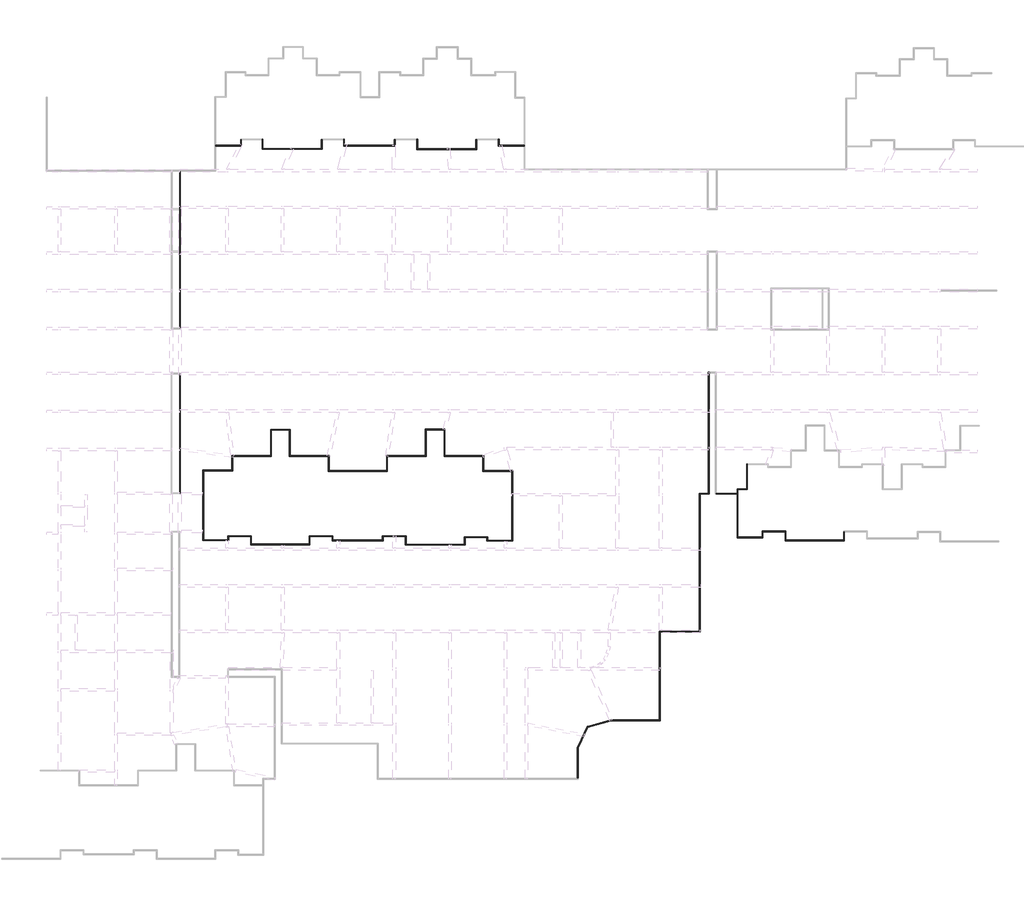
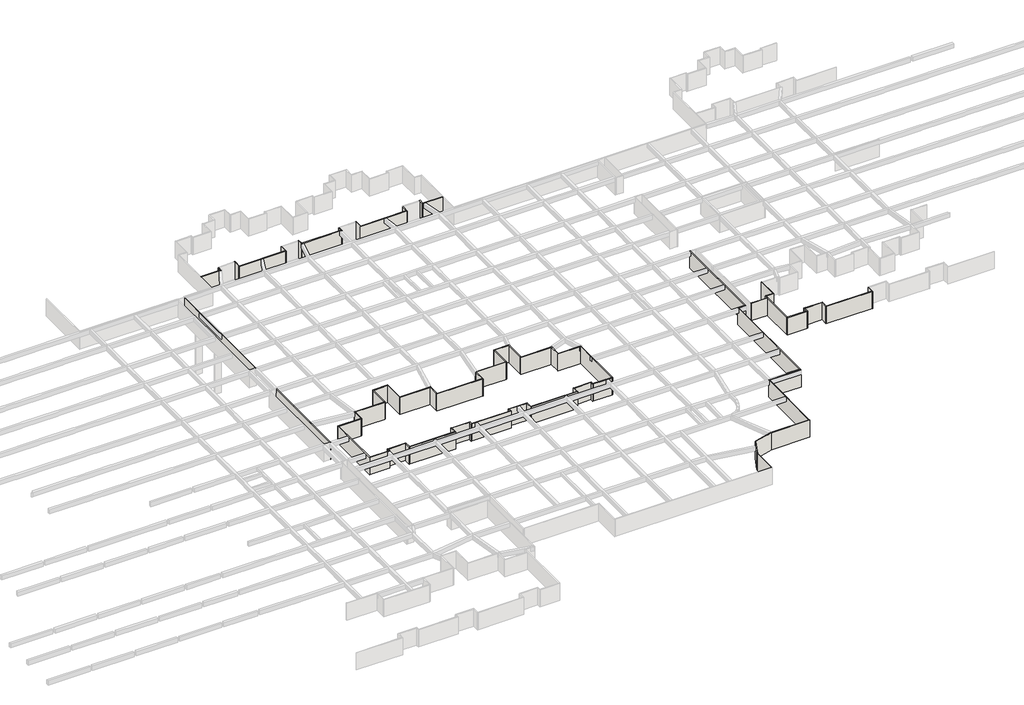
# One storey, part 4 of 16: 70 walls.
"""IFC4 building model written with IfcOpenShell, lengths in millimetres."""

from ifc_helpers import new_model, si_unit, origin, origin_with_axes, place, context, project, spatial, polyline, outline, extrude, faceted_brep, element, save

model = new_model("IFC4")

# Units and contexts
model_context = context("Model", 3, world=origin())
ifc_project = project(units=[si_unit("LENGTHUNIT", "METRE", prefix="MILLI")], contexts=[model_context])

# Site, building, storey
site = spatial("IfcSite", under=ifc_project)
building = spatial("IfcBuilding", under=site)
storey = spatial("IfcBuildingStorey", under=building, Name="户型图", Elevation=0.0)

# Walls
placement = place(None, origin())
element("IfcWall", 1, ObjectType="所有墙体", at=placement, inside=storey, context=model_context, shape_type="Brep", body=[
    faceted_brep([(305606.5285699, -128840.8246701, 0.0), (302019.0558962, -128840.8246701, 0.0), (301899.0558962, -128840.8246701, 0.0), (301899.0558962, -128840.8246701, 3300.0), (302019.0558962, -128840.8246701, 3300.0), (305606.5285699, -128840.8246701, 3300.0), (305606.5285699, -128960.8246701, 0.0), (305606.5285699, -128960.8246701, 3300.0), (301899.0558962, -128960.8246701, 3300.0), (301899.0558962, -128960.8246701, 0.0)], [[[0, 1, 2, 3, 4, 5]], [[6, 7, 8, 9]], [[2, 1, 0, 6, 9]], [[5, 4, 3, 8, 7]], [[0, 5, 7, 6]], [[3, 2, 9, 8]]]),
])
element("IfcWall", 2, ObjectType="所有墙体", at=placement, inside=storey, context=model_context, shape_type="Brep", body=[
    faceted_brep([(302019.0558962, -128840.8246701, 0.0), (302019.0558962, -127937.9986276, 0.0), (302019.0558962, -127937.9986276, 3300.0), (302019.0558962, -128840.8246701, 3300.0), (301899.0558962, -128840.8246701, 0.0), (301899.0558962, -128840.8246701, 3300.0), (301899.0558962, -128057.9986276, 3300.0), (301899.0558962, -127937.9986276, 3300.0), (301899.0558962, -127937.9986276, 0.0), (301899.0558962, -128057.9986276, 0.0)], [[[0, 1, 2, 3]], [[4, 5, 6, 7, 8, 9]], [[1, 0, 4, 9, 8]], [[3, 2, 7, 6, 5]], [[0, 3, 5, 4]], [[2, 1, 8, 7]]]),
])
element("IfcWall", 3, ObjectType="所有墙体", at=placement, inside=storey, context=model_context, shape_type="Brep", body=[
    faceted_brep([(298699.7203632, -128057.9986276, 0.0), (298699.7203632, -129334.4293697, 0.0), (298699.7203632, -129454.4293697, 0.0), (298699.7203632, -129454.4293697, 3300.0), (298699.7203632, -129334.4293697, 3300.0), (298699.7203632, -128057.9986276, 3300.0), (298819.7203632, -128057.9986276, 0.0), (298819.7203632, -128057.9986276, 3300.0), (298819.7203632, -129454.4293697, 3300.0), (298819.7203632, -129454.4293697, 0.0)], [[[0, 1, 2, 3, 4, 5]], [[6, 7, 8, 9]], [[2, 1, 0, 6, 9]], [[5, 4, 3, 8, 7]], [[0, 5, 7, 6]], [[3, 2, 9, 8]]]),
])
element("IfcWall", 4, ObjectType="所有墙体", at=placement, inside=storey, context=model_context, shape_type="Brep", body=[
    faceted_brep([(298699.7203632, -129334.4293697, 0.0), (290319.7203632, -129334.4293697, 0.0), (290199.7203632, -129334.4293697, 0.0), (290199.7203632, -129334.4293697, 3300.0), (290319.7203632, -129334.4293697, 3300.0), (298699.7203632, -129334.4293697, 3300.0), (298699.7203632, -129454.4293697, 0.0), (298699.7203632, -129454.4293697, 3300.0), (290199.7203632, -129454.4293697, 3300.0), (290199.7203632, -129454.4293697, 0.0)], [[[0, 1, 2, 3, 4, 5]], [[6, 7, 8, 9]], [[2, 1, 0, 6, 9]], [[5, 4, 3, 8, 7]], [[0, 5, 7, 6]], [[3, 2, 9, 8]]]),
])
element("IfcWall", 5, ObjectType="所有墙体", at=placement, inside=storey, context=model_context, shape_type="Brep", body=[
    faceted_brep([(290319.7203632, -129334.4293697, 0.0), (290319.7203632, -127937.9986276, 0.0), (290319.7203632, -127937.9986276, 3300.0), (290319.7203632, -129334.4293697, 3300.0), (290199.7203632, -129334.4293697, 0.0), (290199.7203632, -129334.4293697, 3300.0), (290199.7203632, -128057.9986276, 3300.0), (290199.7203632, -127937.9986276, 3300.0), (290199.7203632, -127937.9986276, 0.0), (290199.7203632, -128057.9986276, 0.0)], [[[0, 1, 2, 3]], [[4, 5, 6, 7, 8, 9]], [[1, 0, 4, 9, 8]], [[3, 2, 7, 6, 5]], [[0, 3, 5, 4]], [[2, 1, 8, 7]]]),
])
element("IfcWall", 6, ObjectType="所有墙体", at=placement, inside=storey, context=model_context, shape_type="Brep", body=[
    faceted_brep([(286999.7203632, -128057.9986276, 0.0), (286999.7203632, -128840.8246701, 0.0), (286999.7203632, -128960.8246701, 0.0), (286999.7203632, -128960.8246701, 3300.0), (286999.7203632, -128840.8246701, 3300.0), (286999.7203632, -128057.9986276, 3300.0), (287119.7203632, -128057.9986276, 0.0), (287119.7203632, -128057.9986276, 3300.0), (287119.7203632, -128960.8246701, 3300.0), (287119.7203632, -128960.8246701, 0.0)], [[[0, 1, 2, 3, 4, 5]], [[6, 7, 8, 9]], [[2, 1, 0, 6, 9]], [[5, 4, 3, 8, 7]], [[0, 5, 7, 6]], [[3, 2, 9, 8]]]),
])
element("IfcWall", 7, ObjectType="所有墙体", at=placement, inside=storey, context=model_context, shape_type="Brep", body=[
    faceted_brep([(286999.7203632, -128840.8246701, 0.0), (279819.0680425, -128840.8246701, 0.0), (279699.0680425, -128840.8246701, 0.0), (279699.0680425, -128840.8246701, 3300.0), (279819.0680425, -128840.8246701, 3300.0), (286999.7203632, -128840.8246701, 3300.0), (286999.7203632, -128960.8246701, 0.0), (286999.7203632, -128960.8246701, 3300.0), (279699.0680425, -128960.8246701, 3300.0), (279699.0680425, -128960.8246701, 0.0)], [[[0, 1, 2, 3, 4, 5]], [[6, 7, 8, 9]], [[2, 1, 0, 6, 9]], [[5, 4, 3, 8, 7]], [[0, 5, 7, 6]], [[3, 2, 9, 8]]]),
])
element("IfcWall", 8, ObjectType="所有墙体", at=placement, inside=storey, context=model_context, shape_type="Brep", body=[
    faceted_brep([(279819.0680425, -128840.8246701, 0.0), (279819.0680425, -127937.9986276, 0.0), (279819.0680425, -127937.9986276, 3300.0), (279819.0680425, -128840.8246701, 3300.0), (279699.0680425, -128840.8246701, 0.0), (279699.0680425, -128840.8246701, 3300.0), (279699.0680425, -128057.9986276, 3300.0), (279699.0680425, -127937.9986276, 3300.0), (279699.0680425, -127937.9986276, 0.0), (279699.0680425, -128057.9986276, 0.0)], [[[0, 1, 2, 3]], [[4, 5, 6, 7, 8, 9]], [[1, 0, 4, 9, 8]], [[3, 2, 7, 6, 5]], [[0, 3, 5, 4]], [[2, 1, 8, 7]]]),
])
element("IfcWall", 9, ObjectType="所有墙体", at=placement, inside=storey, context=model_context, shape_type="Brep", body=[
    faceted_brep([(276499.7065412, -128057.9986276, 0.0), (276499.7065412, -129309.6564364, 0.0), (276499.7065412, -129429.6564364, 0.0), (276499.7065412, -129429.6564364, 3300.0), (276499.7065412, -129309.6564364, 3300.0), (276499.7065412, -128057.9986276, 3300.0), (276619.7065412, -128057.9986276, 0.0), (276619.7065412, -128057.9986276, 3300.0), (276619.7065412, -129429.6564364, 3300.0), (276619.7065412, -129429.6564364, 0.0)], [[[0, 1, 2, 3, 4, 5]], [[6, 7, 8, 9]], [[2, 1, 0, 6, 9]], [[5, 4, 3, 8, 7]], [[0, 5, 7, 6]], [[3, 2, 9, 8]]]),
])
element("IfcWall", 10, ObjectType="所有墙体", at=placement, inside=storey, context=model_context, shape_type="Brep", body=[
    faceted_brep([(276499.7065412, -129309.6564364, 0.0), (268118.1706199, -129309.6564364, 0.0), (267998.1706199, -129309.6564364, 0.0), (267998.1706199, -129309.6564364, 3300.0), (268118.1706199, -129309.6564364, 3300.0), (276499.7065412, -129309.6564364, 3300.0), (276499.7065412, -129429.6564364, 0.0), (276499.7065412, -129429.6564364, 3300.0), (267998.1706199, -129429.6564364, 3300.0), (267998.1706199, -129429.6564364, 0.0)], [[[0, 1, 2, 3, 4, 5]], [[6, 7, 8, 9]], [[2, 1, 0, 6, 9]], [[5, 4, 3, 8, 7]], [[0, 5, 7, 6]], [[3, 2, 9, 8]]]),
])
element("IfcWall", 11, ObjectType="所有墙体", at=placement, inside=storey, context=model_context, shape_type="Brep", body=[
    faceted_brep([(268118.1706199, -129309.6564364, 0.0), (268118.1706199, -127937.9986276, 0.0), (268118.1706199, -127937.9986276, 3300.0), (268118.1706199, -129309.6564364, 3300.0), (267998.1706199, -129309.6564364, 0.0), (267998.1706199, -129309.6564364, 3300.0), (267998.1706199, -128057.9986276, 3300.0), (267998.1706199, -127937.9986276, 3300.0), (267998.1706199, -127937.9986276, 0.0), (267998.1706199, -128057.9986276, 0.0)], [[[0, 1, 2, 3]], [[4, 5, 6, 7, 8, 9]], [[1, 0, 4, 9, 8]], [[3, 2, 7, 6, 5]], [[0, 3, 5, 4]], [[2, 1, 8, 7]]]),
])
element("IfcWall", 12, ObjectType="所有墙体", at=placement, inside=storey, context=model_context, shape_type="Brep", body=[
    faceted_brep([(264899.6993188, -128057.9986276, 0.0), (264899.6993188, -128840.8246701, 0.0), (264899.6993188, -128960.8246701, 0.0), (264899.6993188, -128960.8246701, 3300.0), (264899.6993188, -128840.8246701, 3300.0), (264899.6993188, -128057.9986276, 3300.0), (265019.6993188, -128057.9986276, 0.0), (265019.6993188, -128057.9986276, 3300.0), (265019.6993188, -128960.8246701, 3300.0), (265019.6993188, -128960.8246701, 0.0)], [[[0, 1, 2, 3, 4, 5]], [[6, 7, 8, 9]], [[2, 1, 0, 6, 9]], [[5, 4, 3, 8, 7]], [[0, 5, 7, 6]], [[3, 2, 9, 8]]]),
])
element("IfcWall", 13, ObjectType="所有墙体", at=placement, inside=storey, context=model_context, shape_type="SweptSolid", body=[
    extrude(outline(polyline([(261322.7517568, -128840.8246701), (264899.6993188, -128840.8246701), (264899.6993188, -128960.8246701), (261322.7517568, -128960.8246701), (261322.7517568, -128840.8246701)])), origin_with_axes(), (0.0, 0.0, 1.0), 3300.0),
])
element("IfcWall", 14, ObjectType="所有墙体", at=placement, inside=storey, context=model_context, shape_type="Brep", body=[
    faceted_brep([(351498.9314816, -184368.2301972, 0.0), (351498.9314816, -185539.8859396, 0.0), (351498.9314816, -185659.8859396, 0.0), (351498.9314816, -185659.8859396, 3300.0), (351498.9314816, -185539.8859396, 3300.0), (351498.9314816, -184368.2301972, 3300.0), (351618.9314816, -184368.2301972, 0.0), (351618.9314816, -184368.2301972, 3300.0), (351618.9314816, -185659.8859396, 3300.0), (351618.9314816, -185659.8859396, 0.0)], [[[0, 1, 2, 3, 4, 5]], [[6, 7, 8, 9]], [[2, 1, 0, 6, 9]], [[5, 4, 3, 8, 7]], [[0, 5, 7, 6]], [[3, 2, 9, 8]]]),
])
element("IfcWall", 15, ObjectType="所有墙体", at=placement, inside=storey, context=model_context, shape_type="Brep", body=[
    faceted_brep([(351498.9314816, -185539.8859396, 0.0), (343215.8107635, -185539.8859396, 0.0), (343095.8107635, -185539.8859396, 0.0), (343095.8107635, -185539.8859396, 3300.0), (343215.8107635, -185539.8859396, 3300.0), (351498.9314816, -185539.8859396, 3300.0), (351498.9314816, -185659.8859396, 0.0), (351498.9314816, -185659.8859396, 3300.0), (343095.8107635, -185659.8859396, 3300.0), (343095.8107635, -185659.8859396, 0.0)], [[[0, 1, 2, 3, 4, 5]], [[6, 7, 8, 9]], [[2, 1, 0, 6, 9]], [[5, 4, 3, 8, 7]], [[0, 5, 7, 6]], [[3, 2, 9, 8]]]),
])
element("IfcWall", 16, ObjectType="所有墙体", at=placement, inside=storey, context=model_context, shape_type="Brep", body=[
    faceted_brep([(343215.8107635, -185539.8859396, 0.0), (343215.8107635, -184248.2301972, 0.0), (343215.8107635, -184248.2301972, 3300.0), (343215.8107635, -185539.8859396, 3300.0), (343095.8107635, -185539.8859396, 0.0), (343095.8107635, -185539.8859396, 3300.0), (343095.8107635, -184368.2301972, 3300.0), (343095.8107635, -184248.2301972, 3300.0), (343095.8107635, -184248.2301972, 0.0), (343095.8107635, -184368.2301972, 0.0)], [[[0, 1, 2, 3]], [[4, 5, 6, 7, 8, 9]], [[1, 0, 4, 9, 8]], [[3, 2, 7, 6, 5]], [[0, 3, 5, 4]], [[2, 1, 8, 7]]]),
])
element("IfcWall", 17, ObjectType="所有墙体", at=placement, inside=storey, context=model_context, shape_type="Brep", body=[
    faceted_brep([(343095.8107635, -184248.2301972, 0.0), (339799.0678646, -184248.2301972, 0.0), (339799.0678646, -184248.2301972, 3300.0), (343095.8107635, -184248.2301972, 3300.0), (343095.8107635, -184368.2301972, 0.0), (343095.8107635, -184368.2301972, 3300.0), (339919.0678646, -184368.2301972, 3300.0), (339799.0678646, -184368.2301972, 3300.0), (339799.0678646, -184368.2301972, 0.0), (339919.0678646, -184368.2301972, 0.0)], [[[0, 1, 2, 3]], [[4, 5, 6, 7, 8, 9]], [[1, 0, 4, 9, 8]], [[3, 2, 7, 6, 5]], [[0, 3, 5, 4]], [[2, 1, 8, 7]]]),
])
element("IfcWall", 18, ObjectType="所有墙体", at=placement, inside=storey, context=model_context, shape_type="Brep", body=[
    faceted_brep([(339799.0678646, -184368.2301972, 0.0), (339799.0678646, -185110.2860694, 0.0), (339799.0678646, -185230.2860694, 0.0), (339799.0678646, -185230.2860694, 3300.0), (339799.0678646, -185110.2860694, 3300.0), (339799.0678646, -184368.2301972, 3300.0), (339919.0678646, -184368.2301972, 0.0), (339919.0678646, -184368.2301972, 3300.0), (339919.0678646, -185230.2860694, 3300.0), (339919.0678646, -185230.2860694, 0.0)], [[[0, 1, 2, 3, 4, 5]], [[6, 7, 8, 9]], [[2, 1, 0, 6, 9]], [[5, 4, 3, 8, 7]], [[0, 5, 7, 6]], [[3, 2, 9, 8]]]),
])
element("IfcWall", 19, ObjectType="所有墙体", at=placement, inside=storey, context=model_context, shape_type="Brep", body=[
    faceted_brep([(339799.0678646, -185110.2860694, 0.0), (336316.8754953, -185110.2860694, 0.0), (336196.8754953, -185110.2860694, 0.0), (336196.8754953, -185110.2860694, 3300.0), (336316.8754953, -185110.2860694, 3300.0), (339799.0678646, -185110.2860694, 3300.0), (339799.0678646, -185230.2860694, 0.0), (339799.0678646, -185230.2860694, 3300.0), (336196.8754953, -185230.2860694, 3300.0), (336196.8754953, -185230.2860694, 0.0)], [[[0, 1, 2, 3, 4, 5]], [[6, 7, 8, 9]], [[2, 1, 0, 6, 9]], [[5, 4, 3, 8, 7]], [[0, 5, 7, 6]], [[3, 2, 9, 8]]]),
])
element("IfcWall", 20, ObjectType="所有墙体", at=placement, inside=storey, context=model_context, shape_type="Brep", body=[
    faceted_brep([(336316.8754953, -185110.2860694, 0.0), (336316.8754953, -178321.3511104, 0.0), (336316.8754953, -178201.3511104, 0.0), (336316.8754953, -178201.3511104, 3300.0), (336316.8754953, -178321.3511104, 3300.0), (336316.8754953, -185110.2860694, 3300.0), (336196.8754953, -185110.2860694, 0.0), (336196.8754953, -185110.2860694, 3300.0), (336196.8754953, -178965.1471774, 3300.0), (336196.8754953, -178845.1471774, 3300.0), (336196.8754953, -178201.3511104, 3300.0), (336196.8754953, -178201.3511104, 0.0), (336196.8754953, -178845.1471774, 0.0), (336196.8754953, -178965.1471774, 0.0)], [[[0, 1, 2, 3, 4, 5]], [[6, 7, 8, 9, 10, 11, 12, 13]], [[2, 1, 0, 6, 13, 12, 11]], [[5, 4, 3, 10, 9, 8, 7]], [[0, 5, 7, 6]], [[3, 2, 11, 10]]]),
])
element("IfcWall", 21, ObjectType="所有墙体", at=placement, inside=storey, context=model_context, shape_type="Brep", body=[
    faceted_brep([(336316.8754953, -178321.3511104, 0.0), (337684.3582015, -178321.3511104, 0.0), (337684.3582015, -178321.3511104, 3300.0), (336316.8754953, -178321.3511104, 3300.0), (336316.8754953, -178201.3511104, 0.0), (336316.8754953, -178201.3511104, 3300.0), (337564.3582015, -178201.3511104, 3300.0), (337684.3582015, -178201.3511104, 3300.0), (337684.3582015, -178201.3511104, 0.0), (337564.3582015, -178201.3511104, 0.0)], [[[0, 1, 2, 3]], [[4, 5, 6, 7, 8, 9]], [[1, 0, 4, 9, 8]], [[3, 2, 7, 6, 5]], [[0, 3, 5, 4]], [[2, 1, 8, 7]]]),
])
element("IfcWall", 22, ObjectType="所有墙体", at=placement, inside=storey, context=model_context, shape_type="Brep", body=[
    faceted_brep([(337684.3582015, -178201.3511104, 0.0), (337684.3582015, -174724.5990482, 0.0), (337684.3582015, -174604.5990482, 0.0), (337684.3582015, -174604.5990482, 3300.0), (337684.3582015, -174724.5990482, 3300.0), (337684.3582015, -178201.3511104, 3300.0), (337564.3582015, -178201.3511104, 0.0), (337564.3582015, -178201.3511104, 3300.0), (337564.3582015, -174604.5990482, 3300.0), (337564.3582015, -174604.5990482, 0.0)], [[[0, 1, 2, 3, 4, 5]], [[6, 7, 8, 9]], [[2, 1, 0, 6, 9]], [[5, 4, 3, 8, 7]], [[0, 5, 7, 6]], [[3, 2, 9, 8]]]),
])
element("IfcWall", 23, ObjectType="所有墙体", at=placement, inside=storey, context=model_context, shape_type="Brep", body=[
    faceted_brep([(303975.2880408, -185704.0117748, 0.0), (303975.2880408, -175584.0117748, 0.0), (303975.2880408, -175584.0117748, 3300.0), (303975.2880408, -185704.0117748, 3300.0), (303855.2880408, -185704.0117748, 0.0), (303855.2880408, -185704.0117748, 3300.0), (303855.2880408, -185584.0117748, 3300.0), (303855.2880408, -175704.0117748, 3300.0), (303855.2880408, -175584.0117748, 3300.0), (303855.2880408, -175584.0117748, 0.0), (303855.2880408, -175704.0117748, 0.0), (303855.2880408, -185584.0117748, 0.0)], [[[0, 1, 2, 3]], [[4, 5, 6, 7, 8, 9, 10, 11]], [[1, 0, 4, 11, 10, 9]], [[3, 2, 8, 7, 6, 5]], [[2, 1, 9, 8]], [[0, 3, 5, 4]]]),
])
element("IfcWall", 24, ObjectType="所有墙体", at=placement, inside=storey, context=model_context, shape_type="Brep", body=[
    faceted_brep([(303855.2880408, -175584.0117748, 0.0), (299815.2880408, -175584.0117748, 0.0), (299695.2880408, -175584.0117748, 0.0), (299695.2880408, -175584.0117748, 3300.0), (299815.2880408, -175584.0117748, 3300.0), (303855.2880408, -175584.0117748, 3300.0), (303855.2880408, -175704.0117748, 0.0), (303855.2880408, -175704.0117748, 3300.0), (299695.2880408, -175704.0117748, 3300.0), (299695.2880408, -175704.0117748, 0.0)], [[[0, 1, 2, 3, 4, 5]], [[6, 7, 8, 9]], [[2, 1, 0, 6, 9]], [[5, 4, 3, 8, 7]], [[0, 5, 7, 6]], [[3, 2, 9, 8]]]),
])
element("IfcWall", 25, ObjectType="所有墙体", at=placement, inside=storey, context=model_context, shape_type="Brep", body=[
    faceted_brep([(299815.2880408, -175584.0117748, 0.0), (299815.2880408, -173444.0117748, 0.0), (299815.2880408, -173444.0117748, 3300.0), (299815.2880408, -175584.0117748, 3300.0), (299695.2880408, -175584.0117748, 0.0), (299695.2880408, -175584.0117748, 3300.0), (299695.2880408, -173564.0117748, 3300.0), (299695.2880408, -173444.0117748, 3300.0), (299695.2880408, -173444.0117748, 0.0), (299695.2880408, -173564.0117748, 0.0)], [[[0, 1, 2, 3]], [[4, 5, 6, 7, 8, 9]], [[1, 0, 4, 9, 8]], [[3, 2, 7, 6, 5]], [[0, 3, 5, 4]], [[2, 1, 8, 7]]]),
])
element("IfcWall", 26, ObjectType="所有墙体", at=placement, inside=storey, context=model_context, shape_type="Brep", body=[
    faceted_brep([(299695.2880408, -173444.0117748, 0.0), (294238.8289341, -173444.0117748, 0.0), (294118.8289341, -173444.0117748, 0.0), (294118.8289341, -173444.0117748, 3300.0), (294238.8289341, -173444.0117748, 3300.0), (299695.2880408, -173444.0117748, 3300.0), (299695.2880408, -173564.0117748, 0.0), (299695.2880408, -173564.0117748, 3300.0), (294118.8289341, -173564.0117748, 3300.0), (294118.8289341, -173564.0117748, 0.0)], [[[0, 1, 2, 3, 4, 5]], [[6, 7, 8, 9]], [[2, 1, 0, 6, 9]], [[5, 4, 3, 8, 7]], [[0, 5, 7, 6]], [[3, 2, 9, 8]]]),
])
element("IfcWall", 27, ObjectType="所有墙体", at=placement, inside=storey, context=model_context, shape_type="Brep", body=[
    faceted_brep([(294238.8289341, -173444.0117748, 0.0), (294238.8289341, -169623.3600959, 0.0), (294238.8289341, -169623.3600959, 3300.0), (294238.8289341, -173444.0117748, 3300.0), (294118.8289341, -173444.0117748, 0.0), (294118.8289341, -173444.0117748, 3300.0), (294118.8289341, -169743.3600959, 3300.0), (294118.8289341, -169623.3600959, 3300.0), (294118.8289341, -169623.3600959, 0.0), (294118.8289341, -169743.3600959, 0.0)], [[[0, 1, 2, 3]], [[4, 5, 6, 7, 8, 9]], [[1, 0, 4, 9, 8]], [[3, 2, 7, 6, 5]], [[0, 3, 5, 4]], [[2, 1, 8, 7]]]),
])
element("IfcWall", 28, ObjectType="所有墙体", at=placement, inside=storey, context=model_context, shape_type="Brep", body=[
    faceted_brep([(294118.8289341, -169623.3600959, 0.0), (291423.2579583, -169623.3600959, 0.0), (291423.2579583, -169623.3600959, 3300.0), (294118.8289341, -169623.3600959, 3300.0), (294118.8289341, -169743.3600959, 0.0), (294118.8289341, -169743.3600959, 3300.0), (291543.2579583, -169743.3600959, 3300.0), (291423.2579583, -169743.3600959, 3300.0), (291423.2579583, -169743.3600959, 0.0), (291543.2579583, -169743.3600959, 0.0)], [[[0, 1, 2, 3]], [[4, 5, 6, 7, 8, 9]], [[1, 0, 4, 9, 8]], [[3, 2, 7, 6, 5]], [[0, 3, 5, 4]], [[2, 1, 8, 7]]]),
])
element("IfcWall", 29, ObjectType="所有墙体", at=placement, inside=storey, context=model_context, shape_type="Brep", body=[
    faceted_brep([(291423.2579583, -169743.3600959, 0.0), (291423.2579583, -173444.0117748, 0.0), (291423.2579583, -173564.0117748, 0.0), (291423.2579583, -173564.0117748, 3300.0), (291423.2579583, -173444.0117748, 3300.0), (291423.2579583, -169743.3600959, 3300.0), (291543.2579583, -169743.3600959, 0.0), (291543.2579583, -169743.3600959, 3300.0), (291543.2579583, -173564.0117748, 3300.0), (291543.2579583, -173564.0117748, 0.0)], [[[0, 1, 2, 3, 4, 5]], [[6, 7, 8, 9]], [[2, 1, 0, 6, 9]], [[5, 4, 3, 8, 7]], [[0, 5, 7, 6]], [[3, 2, 9, 8]]]),
])
element("IfcWall", 30, ObjectType="所有墙体", at=placement, inside=storey, context=model_context, shape_type="Brep", body=[
    faceted_brep([(291423.2579583, -173444.0117748, 0.0), (285868.9093069, -173444.0117748, 0.0), (285868.9093069, -173444.0117748, 3300.0), (291423.2579583, -173444.0117748, 3300.0), (291423.2579583, -173564.0117748, 0.0), (291423.2579583, -173564.0117748, 3300.0), (285988.9093069, -173564.0117748, 3300.0), (285868.9093069, -173564.0117748, 3300.0), (285868.9093069, -173564.0117748, 0.0), (285988.9093069, -173564.0117748, 0.0)], [[[0, 1, 2, 3]], [[4, 5, 6, 7, 8, 9]], [[1, 0, 4, 9, 8]], [[3, 2, 7, 6, 5]], [[0, 3, 5, 4]], [[2, 1, 8, 7]]]),
])
element("IfcWall", 31, ObjectType="所有墙体", at=placement, inside=storey, context=model_context, shape_type="Brep", body=[
    faceted_brep([(285868.9093069, -173564.0117748, 0.0), (285868.9093069, -175584.0117748, 0.0), (285868.9093069, -175704.0117748, 0.0), (285868.9093069, -175704.0117748, 3300.0), (285868.9093069, -175584.0117748, 3300.0), (285868.9093069, -173564.0117748, 3300.0), (285988.9093069, -173564.0117748, 0.0), (285988.9093069, -173564.0117748, 3300.0), (285988.9093069, -175704.0117748, 3300.0), (285988.9093069, -175704.0117748, 0.0)], [[[0, 1, 2, 3, 4, 5]], [[6, 7, 8, 9]], [[2, 1, 0, 6, 9]], [[5, 4, 3, 8, 7]], [[0, 5, 7, 6]], [[3, 2, 9, 8]]]),
])
element("IfcWall", 32, ObjectType="所有墙体", at=placement, inside=storey, context=model_context, shape_type="Brep", body=[
    faceted_brep([(285868.9093069, -175584.0117748, 0.0), (277626.4306149, -175584.0117748, 0.0), (277506.4306149, -175584.0117748, 0.0), (277506.4306149, -175584.0117748, 3300.0), (277626.4306149, -175584.0117748, 3300.0), (285868.9093069, -175584.0117748, 3300.0), (285868.9093069, -175704.0117748, 0.0), (285868.9093069, -175704.0117748, 3300.0), (277506.4306149, -175704.0117748, 3300.0), (277506.4306149, -175704.0117748, 0.0)], [[[0, 1, 2, 3, 4, 5]], [[6, 7, 8, 9]], [[2, 1, 0, 6, 9]], [[5, 4, 3, 8, 7]], [[0, 5, 7, 6]], [[3, 2, 9, 8]]]),
])
element("IfcWall", 33, ObjectType="所有墙体", at=placement, inside=storey, context=model_context, shape_type="Brep", body=[
    faceted_brep([(277626.4306149, -175584.0117748, 0.0), (277626.4306149, -173424.0117748, 0.0), (277626.4306149, -173424.0117748, 3300.0), (277626.4306149, -175584.0117748, 3300.0), (277506.4306149, -175584.0117748, 0.0), (277506.4306149, -175584.0117748, 3300.0), (277506.4306149, -173544.0117748, 3300.0), (277506.4306149, -173424.0117748, 3300.0), (277506.4306149, -173424.0117748, 0.0), (277506.4306149, -173544.0117748, 0.0)], [[[0, 1, 2, 3]], [[4, 5, 6, 7, 8, 9]], [[1, 0, 4, 9, 8]], [[3, 2, 7, 6, 5]], [[0, 3, 5, 4]], [[2, 1, 8, 7]]]),
])
element("IfcWall", 34, ObjectType="所有墙体", at=placement, inside=storey, context=model_context, shape_type="Brep", body=[
    faceted_brep([(277506.4306149, -173424.0117748, 0.0), (272038.8374301, -173424.0117748, 0.0), (271918.8374301, -173424.0117748, 0.0), (271918.8374301, -173424.0117748, 3300.0), (272038.8374301, -173424.0117748, 3300.0), (277506.4306149, -173424.0117748, 3300.0), (277506.4306149, -173544.0117748, 0.0), (277506.4306149, -173544.0117748, 3300.0), (271918.8374301, -173544.0117748, 3300.0), (271918.8374301, -173544.0117748, 0.0)], [[[0, 1, 2, 3, 4, 5]], [[6, 7, 8, 9]], [[2, 1, 0, 6, 9]], [[5, 4, 3, 8, 7]], [[0, 5, 7, 6]], [[3, 2, 9, 8]]]),
])
element("IfcWall", 35, ObjectType="所有墙体", at=placement, inside=storey, context=model_context, shape_type="Brep", body=[
    faceted_brep([(272038.8374301, -173424.0117748, 0.0), (272038.8374301, -169646.8578212, 0.0), (272038.8374301, -169646.8578212, 3300.0), (272038.8374301, -173424.0117748, 3300.0), (271918.8374301, -173424.0117748, 0.0), (271918.8374301, -173424.0117748, 3300.0), (271918.8374301, -169766.8578212, 3300.0), (271918.8374301, -169646.8578212, 3300.0), (271918.8374301, -169646.8578212, 0.0), (271918.8374301, -169766.8578212, 0.0)], [[[0, 1, 2, 3]], [[4, 5, 6, 7, 8, 9]], [[1, 0, 4, 9, 8]], [[3, 2, 7, 6, 5]], [[0, 3, 5, 4]], [[2, 1, 8, 7]]]),
])
element("IfcWall", 36, ObjectType="所有墙体", at=placement, inside=storey, context=model_context, shape_type="Brep", body=[
    faceted_brep([(271918.8374301, -169646.8578212, 0.0), (269221.9906808, -169646.8578212, 0.0), (269221.9906808, -169646.8578212, 3300.0), (271918.8374301, -169646.8578212, 3300.0), (271918.8374301, -169766.8578212, 0.0), (271918.8374301, -169766.8578212, 3300.0), (269341.9906808, -169766.8578212, 3300.0), (269221.9906808, -169766.8578212, 3300.0), (269221.9906808, -169766.8578212, 0.0), (269341.9906808, -169766.8578212, 0.0)], [[[0, 1, 2, 3]], [[4, 5, 6, 7, 8, 9]], [[1, 0, 4, 9, 8]], [[3, 2, 7, 6, 5]], [[0, 3, 5, 4]], [[2, 1, 8, 7]]]),
])
element("IfcWall", 37, ObjectType="所有墙体", at=placement, inside=storey, context=model_context, shape_type="Brep", body=[
    faceted_brep([(269221.9906808, -169766.8578212, 0.0), (269221.9906808, -173424.0117748, 0.0), (269221.9906808, -173544.0117748, 0.0), (269221.9906808, -173544.0117748, 3300.0), (269221.9906808, -173424.0117748, 3300.0), (269221.9906808, -169766.8578212, 3300.0), (269341.9906808, -169766.8578212, 0.0), (269341.9906808, -169766.8578212, 3300.0), (269341.9906808, -173544.0117748, 3300.0), (269341.9906808, -173544.0117748, 0.0)], [[[0, 1, 2, 3, 4, 5]], [[6, 7, 8, 9]], [[2, 1, 0, 6, 9]], [[5, 4, 3, 8, 7]], [[0, 5, 7, 6]], [[3, 2, 9, 8]]]),
])
element("IfcWall", 38, ObjectType="所有墙体", at=placement, inside=storey, context=model_context, shape_type="Brep", body=[
    faceted_brep([(269221.9906808, -173424.0117748, 0.0), (263668.9231132, -173424.0117748, 0.0), (263668.9231132, -173424.0117748, 3300.0), (269221.9906808, -173424.0117748, 3300.0), (269221.9906808, -173544.0117748, 0.0), (269221.9906808, -173544.0117748, 3300.0), (263788.9231132, -173544.0117748, 3300.0), (263668.9231132, -173544.0117748, 3300.0), (263668.9231132, -173544.0117748, 0.0), (263788.9231132, -173544.0117748, 0.0)], [[[0, 1, 2, 3]], [[4, 5, 6, 7, 8, 9]], [[1, 0, 4, 9, 8]], [[3, 2, 7, 6, 5]], [[0, 3, 5, 4]], [[2, 1, 8, 7]]]),
])
element("IfcWall", 39, ObjectType="所有墙体", at=placement, inside=storey, context=model_context, shape_type="Brep", body=[
    faceted_brep([(263668.9231132, -173544.0117748, 0.0), (263668.9231132, -175524.0117748, 0.0), (263668.9231132, -175644.0117748, 0.0), (263668.9231132, -175644.0117748, 3300.0), (263668.9231132, -175524.0117748, 3300.0), (263668.9231132, -173544.0117748, 3300.0), (263788.9231132, -173544.0117748, 0.0), (263788.9231132, -173544.0117748, 3300.0), (263788.9231132, -175644.0117748, 3300.0), (263788.9231132, -175644.0117748, 0.0)], [[[0, 1, 2, 3, 4, 5]], [[6, 7, 8, 9]], [[2, 1, 0, 6, 9]], [[5, 4, 3, 8, 7]], [[0, 5, 7, 6]], [[3, 2, 9, 8]]]),
])
element("IfcWall", 40, ObjectType="所有墙体", at=placement, inside=storey, context=model_context, shape_type="Brep", body=[
    faceted_brep([(263668.9231132, -175524.0117748, 0.0), (259466.4862994, -175524.0117748, 0.0), (259466.4862994, -175524.0117748, 3300.0), (263668.9231132, -175524.0117748, 3300.0), (263668.9231132, -175644.0117748, 0.0), (263668.9231132, -175644.0117748, 3300.0), (259586.4862994, -175644.0117748, 3300.0), (259466.4862994, -175644.0117748, 3300.0), (259466.4862994, -175644.0117748, 0.0), (259586.4862994, -175644.0117748, 0.0)], [[[0, 1, 2, 3]], [[4, 5, 6, 7, 8, 9]], [[1, 0, 4, 9, 8]], [[3, 2, 7, 6, 5]], [[0, 3, 5, 4]], [[2, 1, 8, 7]]]),
])
element("IfcWall", 41, ObjectType="所有墙体", at=placement, inside=storey, context=model_context, shape_type="Brep", body=[
    faceted_brep([(259466.4862994, -175644.0117748, 0.0), (259466.4862994, -185644.0117748, 0.0), (259466.4862994, -185644.0117748, 3300.0), (259466.4862994, -175644.0117748, 3300.0), (259586.4862994, -175644.0117748, 0.0), (259586.4862994, -175644.0117748, 3300.0), (259586.4862994, -185524.0117748, 3300.0), (259586.4862994, -185644.0117748, 3300.0), (259586.4862994, -185644.0117748, 0.0), (259586.4862994, -185524.0117748, 0.0)], [[[0, 1, 2, 3]], [[4, 5, 6, 7, 8, 9]], [[1, 0, 4, 9, 8]], [[3, 2, 7, 6, 5]], [[0, 3, 5, 4]], [[2, 1, 8, 7]]]),
])
element("IfcWall", 42, ObjectType="所有墙体", at=placement, inside=storey, context=model_context, shape_type="Brep", body=[
    faceted_brep([(259586.4862994, -185644.0117748, 0.0), (263175.329592, -185644.0117748, 0.0), (263175.329592, -185644.0117748, 3300.0), (259586.4862994, -185644.0117748, 3300.0), (259586.4862994, -185524.0117748, 0.0), (259586.4862994, -185524.0117748, 3300.0), (263055.329592, -185524.0117748, 3300.0), (263175.329592, -185524.0117748, 3300.0), (263175.329592, -185524.0117748, 0.0), (263055.329592, -185524.0117748, 0.0)], [[[0, 1, 2, 3]], [[4, 5, 6, 7, 8, 9]], [[1, 0, 4, 9, 8]], [[3, 2, 7, 6, 5]], [[0, 3, 5, 4]], [[2, 1, 8, 7]]]),
])
element("IfcWall", 43, ObjectType="所有墙体", at=placement, inside=storey, context=model_context, shape_type="Brep", body=[
    faceted_brep([(263175.329592, -185524.0117748, 0.0), (263175.329592, -185058.4829368, 0.0), (263175.329592, -184938.4829368, 0.0), (263175.329592, -184938.4829368, 3300.0), (263175.329592, -185058.4829368, 3300.0), (263175.329592, -185524.0117748, 3300.0), (263055.329592, -185524.0117748, 0.0), (263055.329592, -185524.0117748, 3300.0), (263055.329592, -184938.4829368, 3300.0), (263055.329592, -184938.4829368, 0.0)], [[[0, 1, 2, 3, 4, 5]], [[6, 7, 8, 9]], [[2, 1, 0, 6, 9]], [[5, 4, 3, 8, 7]], [[0, 5, 7, 6]], [[3, 2, 9, 8]]]),
])
element("IfcWall", 44, ObjectType="所有墙体", at=placement, inside=storey, context=model_context, shape_type="Brep", body=[
    faceted_brep([(263175.329592, -185058.4829368, 0.0), (266355.9850353, -185058.4829368, 0.0), (266475.9850353, -185058.4829368, 0.0), (266475.9850353, -185058.4829368, 3300.0), (266355.9850353, -185058.4829368, 3300.0), (263175.329592, -185058.4829368, 3300.0), (263175.329592, -184938.4829368, 0.0), (263175.329592, -184938.4829368, 3300.0), (266475.9850353, -184938.4829368, 3300.0), (266475.9850353, -184938.4829368, 0.0)], [[[0, 1, 2, 3, 4, 5]], [[6, 7, 8, 9]], [[2, 1, 0, 6, 9]], [[5, 4, 3, 8, 7]], [[0, 5, 7, 6]], [[3, 2, 9, 8]]]),
])
element("IfcWall", 45, ObjectType="所有墙体", at=placement, inside=storey, context=model_context, shape_type="Brep", body=[
    faceted_brep([(266355.9850353, -185058.4829368, 0.0), (266355.9850353, -186262.1668684, 0.0), (266355.9850353, -186262.1668684, 3300.0), (266355.9850353, -185058.4829368, 3300.0), (266475.9850353, -185058.4829368, 0.0), (266475.9850353, -185058.4829368, 3300.0), (266475.9850353, -186142.1668684, 3300.0), (266475.9850353, -186262.1668684, 3300.0), (266475.9850353, -186262.1668684, 0.0), (266475.9850353, -186142.1668684, 0.0)], [[[0, 1, 2, 3]], [[4, 5, 6, 7, 8, 9]], [[1, 0, 4, 9, 8]], [[3, 2, 7, 6, 5]], [[0, 3, 5, 4]], [[2, 1, 8, 7]]]),
])
element("IfcWall", 46, ObjectType="所有墙体", at=placement, inside=storey, context=model_context, shape_type="Brep", body=[
    faceted_brep([(266475.9850353, -186262.1668684, 0.0), (274874.6470805, -186262.1668684, 0.0), (274874.6470805, -186262.1668684, 3300.0), (266475.9850353, -186262.1668684, 3300.0), (266475.9850353, -186142.1668684, 0.0), (266475.9850353, -186142.1668684, 3300.0), (274754.6470805, -186142.1668684, 3300.0), (274874.6470805, -186142.1668684, 3300.0), (274874.6470805, -186142.1668684, 0.0), (274754.6470805, -186142.1668684, 0.0)], [[[0, 1, 2, 3]], [[4, 5, 6, 7, 8, 9]], [[1, 0, 4, 9, 8]], [[3, 2, 7, 6, 5]], [[0, 3, 5, 4]], [[2, 1, 8, 7]]]),
])
element("IfcWall", 47, ObjectType="所有墙体", at=placement, inside=storey, context=model_context, shape_type="Brep", body=[
    faceted_brep([(274874.6470805, -186142.1668684, 0.0), (274874.6470805, -185062.1668684, 0.0), (274874.6470805, -184942.1668684, 0.0), (274874.6470805, -184942.1668684, 3300.0), (274874.6470805, -185062.1668684, 3300.0), (274874.6470805, -186142.1668684, 3300.0), (274754.6470805, -186142.1668684, 0.0), (274754.6470805, -186142.1668684, 3300.0), (274754.6470805, -184942.1668684, 3300.0), (274754.6470805, -184942.1668684, 0.0)], [[[0, 1, 2, 3, 4, 5]], [[6, 7, 8, 9]], [[2, 1, 0, 6, 9]], [[5, 4, 3, 8, 7]], [[0, 5, 7, 6]], [[3, 2, 9, 8]]]),
])
element("IfcWall", 48, ObjectType="所有墙体", at=placement, inside=storey, context=model_context, shape_type="Brep", body=[
    faceted_brep([(274874.6470805, -185062.1668684, 0.0), (278055.9882089, -185062.1668684, 0.0), (278175.9882089, -185062.1668684, 0.0), (278175.9882089, -185062.1668684, 3300.0), (278055.9882089, -185062.1668684, 3300.0), (274874.6470805, -185062.1668684, 3300.0), (274874.6470805, -184942.1668684, 0.0), (274874.6470805, -184942.1668684, 3300.0), (278175.9882089, -184942.1668684, 3300.0), (278175.9882089, -184942.1668684, 0.0)], [[[0, 1, 2, 3, 4, 5]], [[6, 7, 8, 9]], [[2, 1, 0, 6, 9]], [[5, 4, 3, 8, 7]], [[0, 5, 7, 6]], [[3, 2, 9, 8]]]),
])
element("IfcWall", 49, ObjectType="所有墙体", at=placement, inside=storey, context=model_context, shape_type="Brep", body=[
    faceted_brep([(278055.9882089, -185062.1668684, 0.0), (278055.9882089, -185675.2224684, 0.0), (278055.9882089, -185675.2224684, 3300.0), (278055.9882089, -185062.1668684, 3300.0), (278175.9882089, -185062.1668684, 0.0), (278175.9882089, -185062.1668684, 3300.0), (278175.9882089, -185555.2224684, 3300.0), (278175.9882089, -185675.2224684, 3300.0), (278175.9882089, -185675.2224684, 0.0), (278175.9882089, -185555.2224684, 0.0)], [[[0, 1, 2, 3]], [[4, 5, 6, 7, 8, 9]], [[1, 0, 4, 9, 8]], [[3, 2, 7, 6, 5]], [[0, 3, 5, 4]], [[2, 1, 8, 7]]]),
])
element("IfcWall", 50, ObjectType="所有墙体", at=placement, inside=storey, context=model_context, shape_type="Brep", body=[
    faceted_brep([(278175.9882089, -185675.2224684, 0.0), (285375.3085861, -185675.2224684, 0.0), (285375.3085861, -185675.2224684, 3300.0), (278175.9882089, -185675.2224684, 3300.0), (278175.9882089, -185555.2224684, 0.0), (278175.9882089, -185555.2224684, 3300.0), (285255.3085861, -185555.2224684, 3300.0), (285375.3085861, -185555.2224684, 3300.0), (285375.3085861, -185555.2224684, 0.0), (285255.3085861, -185555.2224684, 0.0)], [[[0, 1, 2, 3]], [[4, 5, 6, 7, 8, 9]], [[1, 0, 4, 9, 8]], [[3, 2, 7, 6, 5]], [[0, 3, 5, 4]], [[2, 1, 8, 7]]]),
])
element("IfcWall", 51, ObjectType="所有墙体", at=placement, inside=storey, context=model_context, shape_type="Brep", body=[
    faceted_brep([(285375.3085861, -185555.2224684, 0.0), (285375.3085861, -185062.1668684, 0.0), (285375.3085861, -184942.1668684, 0.0), (285375.3085861, -184942.1668684, 3300.0), (285375.3085861, -185062.1668684, 3300.0), (285375.3085861, -185555.2224684, 3300.0), (285255.3085861, -185555.2224684, 0.0), (285255.3085861, -185555.2224684, 3300.0), (285255.3085861, -184942.1668684, 3300.0), (285255.3085861, -184942.1668684, 0.0)], [[[0, 1, 2, 3, 4, 5]], [[6, 7, 8, 9]], [[2, 1, 0, 6, 9]], [[5, 4, 3, 8, 7]], [[0, 5, 7, 6]], [[3, 2, 9, 8]]]),
])
element("IfcWall", 52, ObjectType="所有墙体", at=placement, inside=storey, context=model_context, shape_type="Brep", body=[
    faceted_brep([(285375.3085861, -185062.1668684, 0.0), (288555.9947463, -185062.1668684, 0.0), (288675.9947463, -185062.1668684, 0.0), (288675.9947463, -185062.1668684, 3300.0), (288555.9947463, -185062.1668684, 3300.0), (285375.3085861, -185062.1668684, 3300.0), (285375.3085861, -184942.1668684, 0.0), (285375.3085861, -184942.1668684, 3300.0), (288675.9947463, -184942.1668684, 3300.0), (288675.9947463, -184942.1668684, 0.0)], [[[0, 1, 2, 3, 4, 5]], [[6, 7, 8, 9]], [[2, 1, 0, 6, 9]], [[5, 4, 3, 8, 7]], [[0, 5, 7, 6]], [[3, 2, 9, 8]]]),
])
element("IfcWall", 53, ObjectType="所有墙体", at=placement, inside=storey, context=model_context, shape_type="Brep", body=[
    faceted_brep([(288555.9947463, -185062.1668684, 0.0), (288555.9947463, -186286.9397454, 0.0), (288555.9947463, -186286.9397454, 3300.0), (288555.9947463, -185062.1668684, 3300.0), (288675.9947463, -185062.1668684, 0.0), (288675.9947463, -185062.1668684, 3300.0), (288675.9947463, -186166.9397454, 3300.0), (288675.9947463, -186286.9397454, 3300.0), (288675.9947463, -186286.9397454, 0.0), (288675.9947463, -186166.9397454, 0.0)], [[[0, 1, 2, 3]], [[4, 5, 6, 7, 8, 9]], [[1, 0, 4, 9, 8]], [[3, 2, 7, 6, 5]], [[0, 3, 5, 4]], [[2, 1, 8, 7]]]),
])
element("IfcWall", 54, ObjectType="所有墙体", at=placement, inside=storey, context=model_context, shape_type="Brep", body=[
    faceted_brep([(288675.9947463, -186286.9397454, 0.0), (297174.6333207, -186286.9397454, 0.0), (297174.6333207, -186286.9397454, 3300.0), (288675.9947463, -186286.9397454, 3300.0), (288675.9947463, -186166.9397454, 0.0), (288675.9947463, -186166.9397454, 3300.0), (297054.6333207, -186166.9397454, 3300.0), (297174.6333207, -186166.9397454, 3300.0), (297174.6333207, -186166.9397454, 0.0), (297054.6333207, -186166.9397454, 0.0)], [[[0, 1, 2, 3]], [[4, 5, 6, 7, 8, 9]], [[1, 0, 4, 9, 8]], [[3, 2, 7, 6, 5]], [[0, 3, 5, 4]], [[2, 1, 8, 7]]]),
])
element("IfcWall", 55, ObjectType="所有墙体", at=placement, inside=storey, context=model_context, shape_type="Brep", body=[
    faceted_brep([(297174.6333207, -186166.9397454, 0.0), (297174.6333207, -185196.4226478, 0.0), (297174.6333207, -185076.4226478, 0.0), (297174.6333207, -185076.4226478, 3300.0), (297174.6333207, -185196.4226478, 3300.0), (297174.6333207, -186166.9397454, 3300.0), (297054.6333207, -186166.9397454, 0.0), (297054.6333207, -186166.9397454, 3300.0), (297054.6333207, -185076.4226478, 3300.0), (297054.6333207, -185076.4226478, 0.0)], [[[0, 1, 2, 3, 4, 5]], [[6, 7, 8, 9]], [[2, 1, 0, 6, 9]], [[5, 4, 3, 8, 7]], [[0, 5, 7, 6]], [[3, 2, 9, 8]]]),
])
element("IfcWall", 56, ObjectType="所有墙体", at=placement, inside=storey, context=model_context, shape_type="Brep", body=[
    faceted_brep([(297174.6333207, -185196.4226478, 0.0), (300255.8522155, -185196.4226478, 0.0), (300375.8522155, -185196.4226478, 0.0), (300375.8522155, -185196.4226478, 3300.0), (300255.8522155, -185196.4226478, 3300.0), (297174.6333207, -185196.4226478, 3300.0), (297174.6333207, -185076.4226478, 0.0), (297174.6333207, -185076.4226478, 3300.0), (300375.8522155, -185076.4226478, 3300.0), (300375.8522155, -185076.4226478, 0.0)], [[[0, 1, 2, 3, 4, 5]], [[6, 7, 8, 9]], [[2, 1, 0, 6, 9]], [[5, 4, 3, 8, 7]], [[0, 5, 7, 6]], [[3, 2, 9, 8]]]),
])
element("IfcWall", 57, ObjectType="所有墙体", at=placement, inside=storey, context=model_context, shape_type="Brep", body=[
    faceted_brep([(300255.8522155, -185196.4226478, 0.0), (300255.8522155, -185704.0117748, 0.0), (300255.8522155, -185704.0117748, 3300.0), (300255.8522155, -185196.4226478, 3300.0), (300375.8522155, -185196.4226478, 0.0), (300375.8522155, -185196.4226478, 3300.0), (300375.8522155, -185584.0117748, 3300.0), (300375.8522155, -185704.0117748, 3300.0), (300375.8522155, -185704.0117748, 0.0), (300375.8522155, -185584.0117748, 0.0)], [[[0, 1, 2, 3]], [[4, 5, 6, 7, 8, 9]], [[1, 0, 4, 9, 8]], [[3, 2, 7, 6, 5]], [[0, 3, 5, 4]], [[2, 1, 8, 7]]]),
])
element("IfcWall", 58, ObjectType="所有墙体", at=placement, inside=storey, context=model_context, shape_type="SweptSolid", body=[
    extrude(outline(polyline([(303855.2880408, -185704.0117748), (300375.8522155, -185704.0117748), (300375.8522155, -185584.0117748), (303855.2880408, -185584.0117748), (303855.2880408, -185704.0117748)])), origin_with_axes(), (0.0, 0.0, 1.0), 3300.0),
])
element("IfcWall", 59, ObjectType="所有墙体", at=placement, inside=storey, context=model_context, shape_type="Brep", body=[
    faceted_brep([(313389.0126776, -219813.7545432, 0.0), (313389.0126776, -215387.0562229, 0.0), (313389.0126776, -215103.112033, 0.0), (313389.0126776, -215103.112033, 3300.0), (313389.0126776, -215387.0562229, 3300.0), (313389.0126776, -219813.7545432, 3300.0), (313269.0126776, -219813.7545432, 0.0), (313269.0126776, -219813.7545432, 3300.0), (313269.0126776, -215360.4528634, 3300.0), (313269.0126776, -215360.4528634, 0.0)], [[[0, 1, 2, 3, 4, 5]], [[6, 7, 8, 9]], [[2, 1, 0, 6, 9]], [[5, 4, 3, 8, 7]], [[0, 5, 7, 6]], [[3, 2, 9, 8]]]),
])
element("IfcWall", 60, ObjectType="所有墙体", at=placement, inside=storey, context=model_context, shape_type="Brep", body=[
    faceted_brep([(313389.0126776, -215387.0562229, 0.0), (314766.2072007, -212433.6530374, 0.0), (314832.4098758, -212291.6809424, 0.0), (314832.4098758, -212291.6809424, 3300.0), (314766.2072007, -212433.6530374, 3300.0), (313389.0126776, -215387.0562229, 3300.0), (313389.0126776, -215103.112033, 0.0), (313389.0126776, -215103.112033, 3300.0), (314681.0986821, -212332.2246545, 3300.0), (314681.0986821, -212332.2246545, 0.0)], [[[0, 1, 2, 3, 4, 5]], [[6, 7, 8, 9]], [[2, 1, 0, 6, 9]], [[5, 4, 3, 8, 7]], [[0, 5, 7, 6]], [[3, 2, 9, 8]]]),
])
element("IfcWall", 61, ObjectType="所有墙体", at=placement, inside=storey, context=model_context, shape_type="SweptSolid", body=[
    extrude(outline(polyline([(318100.8164668, -211540.1471774), (314766.2072007, -212433.6530374), (314832.4098758, -212291.6809424), (318085.0181671, -211420.1471774), (318100.8164668, -211540.1471774)])), origin_with_axes(), (0.0, 0.0, 1.0), 3300.0),
])
element("IfcWall", 62, ObjectType="所有墙体", at=placement, inside=storey, context=model_context, shape_type="Brep", body=[
    faceted_brep([(318100.8164668, -211540.1471774, 0.0), (325152.9173169, -211540.1471774, 0.0), (325152.9173169, -211540.1471774, 3300.0), (318100.8164668, -211540.1471774, 3300.0), (318085.0181671, -211420.1471774, 0.0), (318085.0181671, -211420.1471774, 3300.0), (325032.9173169, -211420.1471774, 3300.0), (325152.9173169, -211420.1471774, 3300.0), (325152.9173169, -211420.1471774, 0.0), (325032.9173169, -211420.1471774, 0.0)], [[[0, 1, 2, 3]], [[4, 5, 6, 7, 8, 9]], [[1, 0, 4, 9, 8]], [[3, 2, 7, 6, 5]], [[0, 3, 5, 4]], [[2, 1, 8, 7]]]),
])
element("IfcWall", 63, ObjectType="所有墙体", at=placement, inside=storey, context=model_context, shape_type="Brep", body=[
    faceted_brep([(325152.9173169, -211420.1471774, 0.0), (325152.9173169, -198765.1471774, 0.0), (325152.9173169, -198645.1471774, 0.0), (325152.9173169, -198645.1471774, 3300.0), (325152.9173169, -198765.1471774, 3300.0), (325152.9173169, -211420.1471774, 3300.0), (325032.9173169, -211420.1471774, 0.0), (325032.9173169, -211420.1471774, 3300.0), (325032.9173169, -198645.1471774, 3300.0), (325032.9173169, -198645.1471774, 0.0)], [[[0, 1, 2, 3, 4, 5]], [[6, 7, 8, 9]], [[2, 1, 0, 6, 9]], [[5, 4, 3, 8, 7]], [[0, 5, 7, 6]], [[3, 2, 9, 8]]]),
])
element("IfcWall", 64, ObjectType="所有墙体", at=placement, inside=storey, context=model_context, shape_type="Brep", body=[
    faceted_brep([(325152.9173169, -198765.1471774, 0.0), (330913.757676, -198765.1471774, 0.0), (330913.757676, -198765.1471774, 3300.0), (325152.9173169, -198765.1471774, 3300.0), (325152.9173169, -198645.1471774, 0.0), (325152.9173169, -198645.1471774, 3300.0), (330793.757676, -198645.1471774, 3300.0), (330913.757676, -198645.1471774, 3300.0), (330913.757676, -198645.1471774, 0.0), (330793.757676, -198645.1471774, 0.0)], [[[0, 1, 2, 3]], [[4, 5, 6, 7, 8, 9]], [[1, 0, 4, 9, 8]], [[3, 2, 7, 6, 5]], [[0, 3, 5, 4]], [[2, 1, 8, 7]]]),
])
element("IfcWall", 65, ObjectType="所有墙体", at=placement, inside=storey, context=model_context, shape_type="Brep", body=[
    faceted_brep([(330913.757676, -198645.1471774, 0.0), (330913.757676, -178965.1471774, 0.0), (330913.757676, -178845.1471774, 0.0), (330913.757676, -178845.1471774, 3300.0), (330913.757676, -178965.1471774, 3300.0), (330913.757676, -198645.1471774, 3300.0), (330793.757676, -198645.1471774, 0.0), (330793.757676, -198645.1471774, 3300.0), (330793.757676, -178845.1471774, 3300.0), (330793.757676, -178845.1471774, 0.0)], [[[0, 1, 2, 3, 4, 5]], [[6, 7, 8, 9]], [[2, 1, 0, 6, 9]], [[5, 4, 3, 8, 7]], [[0, 5, 7, 6]], [[3, 2, 9, 8]]]),
])
element("IfcWall", 66, ObjectType="所有墙体", at=placement, inside=storey, context=model_context, shape_type="Brep", body=[
    faceted_brep([(330913.757676, -178965.1471774, 0.0), (332213.7576761, -178965.1471774, 0.0), (332213.7576761, -178965.1471774, 3300.0), (330913.757676, -178965.1471774, 3300.0), (330913.757676, -178845.1471774, 0.0), (330913.757676, -178845.1471774, 3300.0), (332093.7576761, -178845.1471774, 3300.0), (332213.7576761, -178845.1471774, 3300.0), (332213.7576761, -178845.1471774, 0.0), (332093.7576761, -178845.1471774, 0.0)], [[[0, 1, 2, 3]], [[4, 5, 6, 7, 8, 9]], [[1, 0, 4, 9, 8]], [[3, 2, 7, 6, 5]], [[0, 3, 5, 4]], [[2, 1, 8, 7]]]),
])
element("IfcWall", 67, ObjectType="所有墙体", at=placement, inside=storey, context=model_context, shape_type="Brep", body=[
    faceted_brep([(332213.7576761, -178845.1471774, 0.0), (332213.7576761, -161565.1471774, 0.0), (332213.7576761, -161445.1471774, 0.0), (332213.7576761, -161445.1471774, 3300.0), (332213.7576761, -161565.1471774, 3300.0), (332213.7576761, -178845.1471774, 3300.0), (332093.7576761, -178845.1471774, 0.0), (332093.7576761, -178845.1471774, 3300.0), (332093.7576761, -161445.1471774, 3300.0), (332093.7576761, -161445.1471774, 0.0)], [[[0, 1, 2, 3, 4, 5]], [[6, 7, 8, 9]], [[2, 1, 0, 6, 9]], [[5, 4, 3, 8, 7]], [[0, 5, 7, 6]], [[3, 2, 9, 8]]]),
])
element("IfcWall", 68, ObjectType="所有墙体", at=placement, inside=storey, context=model_context, shape_type="SweptSolid", body=[
    extrude(outline(polyline([(336196.8754953, -178965.1471774), (333213.7576761, -178965.1471774), (333213.7576761, -178845.1471774), (336196.8754953, -178845.1471774), (336196.8754953, -178965.1471774)])), origin_with_axes(), (0.0, 0.0, 1.0), 3300.0),
])
element("IfcWall", 69, ObjectType="所有墙体", at=placement, inside=storey, context=model_context, shape_type="SweptSolid", body=[
    extrude(outline(polyline([(256263.757676, -132556.8999905), (256263.757676, -155098.1403142), (256143.757676, -155098.1403142), (256143.757676, -132556.8999905), (256263.757676, -132556.8999905)])), origin_with_axes(), (0.0, 0.0, 1.0), 3300.0),
])
element("IfcWall", 70, ObjectType="所有墙体", at=placement, inside=storey, context=model_context, shape_type="Brep", body=[
    faceted_brep([(256143.757676, -161686.0461868, 0.0), (256143.757676, -178766.0461868, 0.0), (256143.757676, -178886.0461868, 0.0), (256143.757676, -178886.0461868, 3300.0), (256143.757676, -178766.0461868, 3300.0), (256143.757676, -161686.0461868, 3300.0), (256263.757676, -161686.0461868, 0.0), (256263.757676, -161686.0461868, 3300.0), (256263.757676, -178886.0461868, 3300.0), (256263.757676, -178886.0461868, 0.0)], [[[0, 1, 2, 3, 4, 5]], [[6, 7, 8, 9]], [[2, 1, 0, 6, 9]], [[5, 4, 3, 8, 7]], [[0, 5, 7, 6]], [[3, 2, 9, 8]]]),
])

save(model, "model.ifc")

# Revit data of these elements
# Type "所有墙体"
#   Layers, outside or top first: 120 mm "默认" (function 1)
# Elements 1, 2, 3, 4, 5, 6, 7, 8, 9, 10, 11, 12, 13, 14, 15, 16, 17, 18, 19, 20, 21, 22, 23, 24, 25, 26, 27, 28, 29, 30, 31, 32, 33, 34, 35, 36, 37, 38, 39, 40, 41, 42, 43, 44, 45, 46, 47, 48, 49, 50, 51, 52, 53, 54, 55, 56, 57, 58, 59, 60, 61, 62, 63, 64, 65, 66, 67, 68, 69, 70 (IfcWall, "所有墙体")
#   Top Offset = 0 mm
#   Base Offset = 0 mm
#   wall height = 3300 mm
#   Phase Created = 新构造
#   Base Constraint = 户型图
#   Top Constraint = 层高
#   Materials on its faces: "默认"
# Materials
#   "默认": class "其他", colour RGB 192 192 192, transparency 0, Cost = 0
